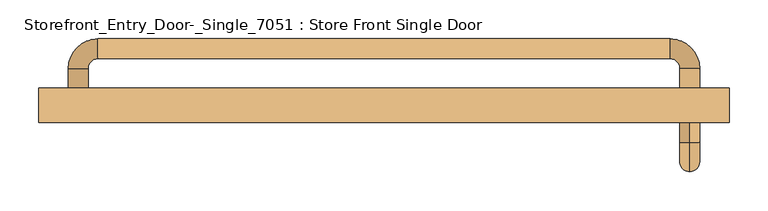
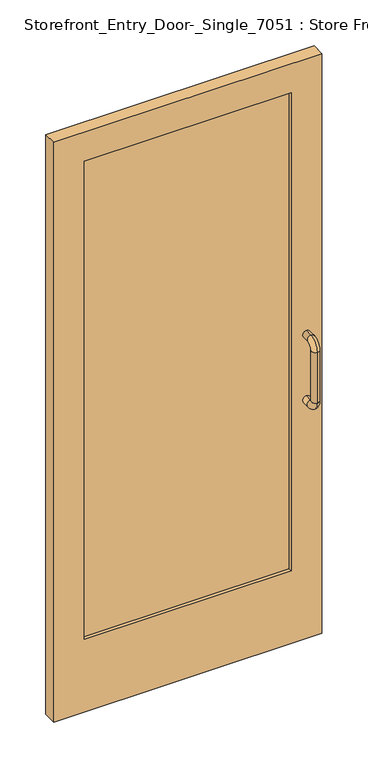
"""IFC4 building model written with IfcOpenShell, lengths in millimetres: door geometry, Storefront_Entry_Door-_Single_7051 : Store Front Single Door."""

from ifc_helpers import new_model, si_unit, point, frame, origin, place, context, project, spatial, polyline, circle_curve, ellipse_curve, trimmed, outline, extrude, source, transform, mapped, element, save
from ifc_brep_helpers import plane_surface, cylinder_surface, revolved_surface, advanced_brep


def storefront_entry_door_single_7051_store_front_single_door_6e28b635(model_context):
    return source(origin(), model_context, "Body", "SolidModel", [
        advanced_brep(
        [(393.7, -50.8, 1054.1), (393.7, -50.8, 1079.5), (393.7, -76.2, 1079.5), (393.7, -76.2, 1054.1), (393.7, -114.3, 1041.4), (393.7, -88.9, 1041.4), (393.7, -114.3, 863.6), (393.7, -88.9, 863.6), (393.7, -76.2, 825.5), (393.7, -76.2, 850.9), (393.7, -50.8, 850.9), (393.7, -50.8, 825.5)],
        [
            (0, 1, circle_curve(frame((393.7, -50.8, 1066.8), z_axis=(0.0, 1.0, 0.0), x_axis=(0.0, 0.0, 1.0)), 12.7)),
            (1, 0, circle_curve(frame((393.7, -50.8, 1066.8), z_axis=(0.0, 1.0, 0.0), x_axis=(0.0, 0.0, 1.0)), 12.7)),
            (1, 2),
            (2, 3, circle_curve(frame((393.7, -76.2, 1066.8), z_axis=(0.0, 1.0, 0.0), x_axis=(0.0, 0.0, 1.0)), 12.7)),
            (3, 0),
            (3, 2, circle_curve(frame((393.7, -76.2, 1066.8), z_axis=(0.0, 1.0, 0.0), x_axis=(0.0, 0.0, 1.0)), 12.7)),
            (4, 5, circle_curve(frame((393.7, -101.6, 1041.4), z_axis=(0.0, 0.0, 1.0), x_axis=(0.0, -1.0, 0.0)), 12.7)),
            (5, 3, circle_curve(frame((393.7, -76.2, 1041.4), z_axis=(-1.0, 0.0, 0.0), x_axis=(0.0, 0.0, 1.0)), 12.7)),
            (2, 4, circle_curve(frame((393.7, -76.2, 1041.4), z_axis=(1.0, 0.0, 0.0), x_axis=(0.0, 0.0, 1.0)), 38.1)),
            (5, 4, circle_curve(frame((393.7, -101.6, 1041.4), z_axis=(0.0, 0.0, 1.0), x_axis=(0.0, -1.0, 0.0)), 12.7)),
            (4, 6),
            (6, 7, circle_curve(frame((393.7, -101.6, 863.6), z_axis=(0.0, 0.0, 1.0), x_axis=(0.0, -1.0, 0.0)), 12.7)),
            (7, 5),
            (7, 6, circle_curve(frame((393.7, -101.6, 863.6), z_axis=(0.0, 0.0, 1.0), x_axis=(0.0, -1.0, 0.0)), 12.7)),
            (8, 9, circle_curve(frame((393.7, -76.2, 838.2), z_axis=(0.0, -1.0, 0.0), x_axis=(0.0, 0.0, -1.0)), 12.7)),
            (9, 7, circle_curve(frame((393.7, -76.2, 863.6), z_axis=(-1.0, 0.0, 0.0), x_axis=(0.0, -1.0, 0.0)), 12.7)),
            (6, 8, circle_curve(frame((393.7, -76.2, 863.6), z_axis=(1.0, 0.0, 0.0), x_axis=(0.0, -1.0, 0.0)), 38.1)),
            (9, 8, circle_curve(frame((393.7, -76.2, 838.2), z_axis=(0.0, -1.0, 0.0), x_axis=(0.0, 0.0, -1.0)), 12.7)),
            (10, 11, circle_curve(frame((393.7, -50.8, 838.2), z_axis=(0.0, 1.0, 0.0), x_axis=(0.0, 0.0, -1.0)), 12.7)),
            (11, 10, circle_curve(frame((393.7, -50.8, 838.2), z_axis=(0.0, 1.0, 0.0), x_axis=(0.0, 0.0, -1.0)), 12.7)),
            (8, 11),
            (10, 9),
        ],
        [
            plane_surface(frame((393.7, -50.8, 1066.8), z_axis=(0.0, 1.0, 0.0), x_axis=(1.0, 0.0, 0.0))),
            cylinder_surface(frame((393.7, -50.8, 1066.8), z_axis=(0.0, 1.0, 0.0), x_axis=(0.0, 0.0, 1.0)), 12.7),
            revolved_surface(trimmed(ellipse_curve(frame((393.7, -76.2, 1066.8), z_axis=(0.0, -1.0, 0.0), x_axis=(0.0, 0.0, 1.0)), 12.7, 12.7), [point((393.7, -76.2, 1054.1))], [point((393.7, -76.2, 1079.5))], True, "CARTESIAN"), (393.7, -76.2, 1041.4), (-1.0, 0.0, 0.0)),
            revolved_surface(trimmed(ellipse_curve(frame((393.7, -76.2, 1066.8), z_axis=(0.0, -1.0, 0.0), x_axis=(0.0, 0.0, 1.0)), 12.7, 12.7), [point((393.7, -76.2, 1079.5))], [point((393.7, -76.2, 1054.1))], True, "CARTESIAN"), (393.7, -76.2, 1041.4), (-1.0, 0.0, 0.0)),
            cylinder_surface(frame((393.7, -101.6, 1041.4), z_axis=(0.0, 0.0, 1.0), x_axis=(0.0, -1.0, 0.0)), 12.7),
            revolved_surface(trimmed(ellipse_curve(frame((393.7, -101.6, 863.6), z_axis=(0.0, 0.0, -1.0), x_axis=(0.0, -1.0, 0.0)), 12.7, 12.7), [point((393.7, -88.9, 863.6))], [point((393.7, -114.3, 863.6))], True, "CARTESIAN"), (393.7, -76.2, 863.6), (-1.0, 0.0, 0.0)),
            revolved_surface(trimmed(ellipse_curve(frame((393.7, -101.6, 863.6), z_axis=(0.0, 0.0, -1.0), x_axis=(0.0, -1.0, 0.0)), 12.7, 12.7), [point((393.7, -114.3, 863.6))], [point((393.7, -88.9, 863.6))], True, "CARTESIAN"), (393.7, -76.2, 863.6), (-1.0, 0.0, 0.0)),
            plane_surface(frame((393.7, -50.8, 838.2), z_axis=(0.0, 1.0, 0.0), x_axis=(1.0, 0.0, 0.0))),
            cylinder_surface(frame((393.7, -76.2, 838.2), z_axis=(0.0, -1.0, 0.0), x_axis=(0.0, 0.0, -1.0)), 12.7),
        ],
        [
            (0, [[1, 2]]),
            (1, [[3, 4, 5, -2]]),
            (1, [[-5, 6, -3, -1]]),
            (2, [[7, 8, -4, 9]]),
            (3, [[10, -9, -6, -8]]),
            (4, [[11, 12, 13, -7]]),
            (4, [[-13, 14, -11, -10]]),
            (5, [[15, 16, -12, 17]]),
            (6, [[18, -17, -14, -16]]),
            (7, [[19, 20]]),
            (8, [[21, -19, 22, -15]]),
            (8, [[-22, -20, -21, -18]]),
        ],
    ),
        advanced_brep(
        [(381.0, -6.35, 1066.8), (406.4, -6.35, 1066.8), (406.4, 19.05, 1066.8), (381.0, 19.05, 1066.8), (368.3, 57.15, 1066.8), (368.3, 31.75, 1066.8), (-368.3, 57.15, 1066.8), (-368.3, 31.75, 1066.8), (-406.4, 19.05, 1066.8), (-381.0, 19.05, 1066.8), (-381.0, -6.35, 1066.8), (-406.4, -6.35, 1066.8)],
        [
            (0, 1, circle_curve(frame((393.7, -6.35, 1066.8), z_axis=(0.0, -1.0, 0.0), x_axis=(1.0, 0.0, 0.0)), 12.7)),
            (1, 0, circle_curve(frame((393.7, -6.35, 1066.8), z_axis=(0.0, -1.0, 0.0), x_axis=(1.0, 0.0, 0.0)), 12.7)),
            (1, 2),
            (2, 3, circle_curve(frame((393.7, 19.05, 1066.8), z_axis=(0.0, -1.0, 0.0), x_axis=(1.0, 0.0, 0.0)), 12.7)),
            (3, 0),
            (3, 2, circle_curve(frame((393.7, 19.05, 1066.8), z_axis=(0.0, -1.0, 0.0), x_axis=(1.0, 0.0, 0.0)), 12.7)),
            (4, 5, circle_curve(frame((368.3, 44.45, 1066.8), z_axis=(1.0, 0.0, 0.0), x_axis=(0.0, 1.0, 0.0)), 12.7)),
            (5, 3, circle_curve(frame((368.3, 19.05, 1066.8), z_axis=(0.0, 0.0, -1.0), x_axis=(1.0, 0.0, 0.0)), 12.7)),
            (2, 4, circle_curve(frame((368.3, 19.05, 1066.8), z_axis=(0.0, 0.0, 1.0), x_axis=(1.0, 0.0, 0.0)), 38.1)),
            (5, 4, circle_curve(frame((368.3, 44.45, 1066.8), z_axis=(1.0, 0.0, 0.0), x_axis=(0.0, 1.0, 0.0)), 12.7)),
            (4, 6),
            (6, 7, circle_curve(frame((-368.3, 44.45, 1066.8), z_axis=(1.0, 0.0, 0.0), x_axis=(0.0, 1.0, 0.0)), 12.7)),
            (7, 5),
            (7, 6, circle_curve(frame((-368.3, 44.45, 1066.8), z_axis=(1.0, 0.0, 0.0), x_axis=(0.0, 1.0, 0.0)), 12.7)),
            (8, 9, circle_curve(frame((-393.7, 19.05, 1066.8), z_axis=(0.0, 1.0, 0.0), x_axis=(-1.0, 0.0, 0.0)), 12.7)),
            (9, 7, circle_curve(frame((-368.3, 19.05, 1066.8), z_axis=(0.0, 0.0, -1.0), x_axis=(0.0, 1.0, 0.0)), 12.7)),
            (6, 8, circle_curve(frame((-368.3, 19.05, 1066.8), z_axis=(0.0, 0.0, 1.0), x_axis=(0.0, 1.0, 0.0)), 38.1)),
            (9, 8, circle_curve(frame((-393.7, 19.05, 1066.8), z_axis=(0.0, 1.0, 0.0), x_axis=(-1.0, 0.0, 0.0)), 12.7)),
            (10, 11, circle_curve(frame((-393.7, -6.35, 1066.8), z_axis=(0.0, -1.0, 0.0), x_axis=(-1.0, 0.0, 0.0)), 12.7)),
            (11, 10, circle_curve(frame((-393.7, -6.35, 1066.8), z_axis=(0.0, -1.0, 0.0), x_axis=(-1.0, 0.0, 0.0)), 12.7)),
            (8, 11),
            (10, 9),
        ],
        [
            plane_surface(frame((393.7, -6.35, 1066.8), z_axis=(0.0, -1.0, 0.0), x_axis=(0.0, 0.0, 1.0))),
            cylinder_surface(frame((393.7, -6.35, 1066.8), z_axis=(0.0, -1.0, 0.0), x_axis=(1.0, 0.0, 0.0)), 12.7),
            revolved_surface(trimmed(ellipse_curve(frame((393.7, 19.05, 1066.8), z_axis=(0.0, 1.0, 0.0), x_axis=(1.0, 0.0, 0.0)), 12.7, 12.7), [point((381.0, 19.05, 1066.8))], [point((406.4, 19.05, 1066.8))], True, "CARTESIAN"), (368.3, 19.05, 1066.8), (0.0, 0.0, -1.0)),
            revolved_surface(trimmed(ellipse_curve(frame((393.7, 19.05, 1066.8), z_axis=(0.0, 1.0, 0.0), x_axis=(1.0, 0.0, 0.0)), 12.7, 12.7), [point((406.4, 19.05, 1066.8))], [point((381.0, 19.05, 1066.8))], True, "CARTESIAN"), (368.3, 19.05, 1066.8), (0.0, 0.0, -1.0)),
            cylinder_surface(frame((368.3, 44.45, 1066.8), z_axis=(1.0, 0.0, 0.0), x_axis=(0.0, 1.0, 0.0)), 12.7),
            revolved_surface(trimmed(ellipse_curve(frame((-368.3, 44.45, 1066.8), z_axis=(-1.0, 0.0, 0.0), x_axis=(0.0, 1.0, 0.0)), 12.7, 12.7), [point((-368.3, 31.75, 1066.8))], [point((-368.3, 57.15, 1066.8))], True, "CARTESIAN"), (-368.3, 19.05, 1066.8), (0.0, 0.0, -1.0)),
            revolved_surface(trimmed(ellipse_curve(frame((-368.3, 44.45, 1066.8), z_axis=(-1.0, 0.0, 0.0), x_axis=(0.0, 1.0, 0.0)), 12.7, 12.7), [point((-368.3, 57.15, 1066.8))], [point((-368.3, 31.75, 1066.8))], True, "CARTESIAN"), (-368.3, 19.05, 1066.8), (0.0, 0.0, -1.0)),
            plane_surface(frame((-393.7, -6.35, 1066.8), z_axis=(0.0, -1.0, 0.0), x_axis=(0.0, 0.0, 1.0))),
            cylinder_surface(frame((-393.7, 19.05, 1066.8), z_axis=(0.0, 1.0, 0.0), x_axis=(-1.0, 0.0, 0.0)), 12.7),
        ],
        [
            (0, [[1, 2]]),
            (1, [[3, 4, 5, -2]]),
            (1, [[-5, 6, -3, -1]]),
            (2, [[7, 8, -4, 9]]),
            (3, [[10, -9, -6, -8]]),
            (4, [[11, 12, 13, -7]]),
            (4, [[-13, 14, -11, -10]]),
            (5, [[15, 16, -12, 17]]),
            (6, [[18, -17, -14, -16]]),
            (7, [[19, 20]]),
            (8, [[21, -19, 22, -15]]),
            (8, [[-22, -20, -21, -18]]),
        ],
    ),
        extrude(outline(polyline([(342.9, -19.05), (342.9, -38.1), (-342.9, -38.1), (-342.9, -19.05), (342.9, -19.05)])), frame((0.0, 0.0, 254.0), z_axis=(0.0, 0.0, 1.0), x_axis=(1.0, 0.0, 0.0)), (0.0, 0.0, 1.0), 1676.4),
        extrude(outline(polyline([(2032.0, 444.5), (2032.0, -444.5), (0.0, -444.5), (0.0, 444.5), (2032.0, 444.5)]), holes=[polyline([(1930.4, -342.9), (1930.4, 342.9), (254.0, 342.9), (254.0, -342.9), (1930.4, -342.9)])]), frame((0.0, -50.8, 0.0), z_axis=(0.0, 1.0, 0.0), x_axis=(0.0, 0.0, 1.0)), (0.0, 0.0, 1.0), 44.45),
    ])


if __name__ == "__main__":
    model = new_model("IFC4")
    model_context = context("Model", 3, world=origin())
    ifc_project = project(units=[si_unit("LENGTHUNIT", "METRE", prefix="MILLI")], contexts=[model_context])
    site = spatial("IfcSite", under=ifc_project)
    building = spatial("IfcBuilding", under=site)
    placement = place(None, origin())
    storefront_entry_door_single_7051_store_front_single_door_shape = storefront_entry_door_single_7051_store_front_single_door_6e28b635(model_context)
    element("IfcDoor", 1, ObjectType="Storefront_Entry_Door-_Single_7051 : Store Front Single Door", at=placement, inside=building, context=model_context, shape_type="MappedRepresentation", body=[
        mapped(storefront_entry_door_single_7051_store_front_single_door_shape, transform((0.0, 0.0, 0.0), x_axis=(1.0, 0.0, 0.0), y_axis=(0.0, 1.0, 0.0), z_axis=(0.0, 0.0, 1.0))),
    ])
    save(model, "model.ifc")

# Revit data of these elements
# Type "Storefront_Entry_Door-_Single_7051 : Store Front Single Door"
#   Type Mark = "19"
#   Assembly Code = "B2030110"
#   Analytic Construction = "<None>"
#   Top Rail = 0' - 4"
#   Side Rail = 0' - 4"
#   Reporting Width [instance default] = 4' - 2"
#   Rail Height AFF = 3' - 6"
#   Offset = 0' - 2"
#   Door Width [instance default] = 4' - 2"
#   Bottom Rail Width = 0' - 10"
#   Material = accent 1
#   Glazing Material = Glass
#   Function = (empty or 0)
# Element 1 (IfcDoor, "Storefront_Entry_Door-_Single_7051 : Store Front Single Door")
#   Reporting Width = 2' - 11"
#   Door Width = 2' - 11"
#   Materials on its faces: "accent 1", "Glass"
# Materials
#   "accent 1": class "Generic", colour RGB 92 104 51, transparency 0, Cost = 0
#   "Glass": class "Glass", colour RGB 236 240 239, transparency 0.85, Description = "Soda Lime Glass", Cost = 0
